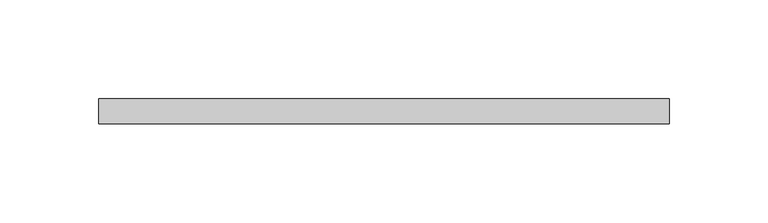
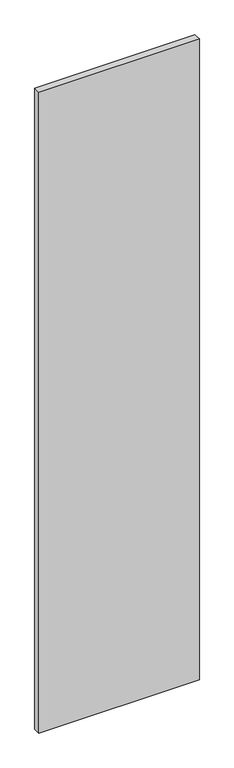
"""IFC4 building model written with IfcOpenShell, lengths in millimetres: proxy geometry, Inner panel:Inner panel:1:Inner panel:1 : Inner panel:Inner panel:300324:300043:Inner panel:1:Inner panel:1 : Inner panel:Inner panel:300324:300043 : Inner panel:Inner panel:1:Inner panel:1 : Inner panel:Inner panel:300324:300043:30 : Inner panel:Inner panel:1:Inner panel:1 : Inner panel:Inner panel:300324:300043:Inner panel:1:Inner panel:1 : Inner panel:Inner panel:300324:300043 : Inner panel:Inner panel:1:Inner panel:1 : Inner panel:Inner panel:300324:300043:300031."""

from ifc_helpers import new_model, si_unit, frame, origin, place, context, project, spatial, polyline, outline, extrude, source, transform, mapped, element, save


def generic_models_07b13941(model_context):
    return source(origin(), model_context, "Body", "SweptSolid", [
        extrude(outline(polyline([(560352.9617239, -579000.6913841), (560641.8867239, -579000.6913841), (560641.8867239, -579013.3913841), (560352.9617239, -579013.3913841), (560352.9617239, -579000.6913841)])), frame((0.0, 0.0, 4946.65), z_axis=(0.0, 0.0, 1.0), x_axis=(1.0, 0.0, 0.0)), (0.0, 0.0, 1.0), 1219.2),
    ])


if __name__ == "__main__":
    model = new_model("IFC4")
    model_context = context("Model", 3, world=origin())
    ifc_project = project(units=[si_unit("LENGTHUNIT", "METRE", prefix="MILLI")], contexts=[model_context])
    site = spatial("IfcSite", under=ifc_project)
    building = spatial("IfcBuilding", under=site)
    placement = place(None, origin())
    generic_models_shape = generic_models_07b13941(model_context)
    element("IfcBuildingElementProxy", 1, Name="Inner panel:Inner panel:1:Inner panel:1 : Inner panel:Inner panel:300324:300043:Inner panel:1:Inner panel:1 : Inner panel:Inner panel:300324:300043 : Inner panel:Inner panel:1:Inner panel:1 : Inner panel:Inner panel:300324:300043:30 : Inner panel:Inner panel:1:Inner panel:1 : Inner panel:Inner panel:300324:300043:Inner panel:1:Inner panel:1 : Inner panel:Inner panel:300324:300043 : Inner panel:Inner panel:1:Inner panel:1 : Inner panel:Inner panel:300324:300043:300031", ObjectType="Inner panel:Inner panel:1:Inner panel:1 : Inner panel:Inner panel:300324:300043:Inner panel:1:Inner panel:1 : Inner panel:Inner panel:300324:300043 : Inner panel:Inner panel:1:Inner panel:1 : Inner panel:Inner panel:300324:300043:30 : Inner panel:Inner panel:1:Inner panel:1 : Inner panel:Inner panel:300324:300043:Inner panel:1:Inner panel:1 : Inner panel:Inner panel:300324:300043 : Inner panel:Inner panel:1:Inner panel:1 : Inner panel:Inner panel:300324:300043:300031", at=placement, inside=building, context=model_context, shape_type="MappedRepresentation", body=[
        mapped(generic_models_shape, transform((0.0, 0.0, 0.0), x_axis=(1.0, 0.0, 0.0), y_axis=(0.0, 1.0, 0.0), z_axis=(0.0, 0.0, 1.0))),
    ])
    save(model, "model.ifc")

# Revit data of these elements
# Type "Inner panel:Inner panel:1:Inner panel:1 : Inner panel:Inner panel:300324:300043:Inner panel:1:Inner panel:1 : Inner panel:Inner panel:300324:300043 : Inner panel:Inner panel:1:Inner panel:1 : Inner panel:Inner panel:300324:300043:30 : Inner panel:Inner panel:1:Inner panel:1 : Inner panel:Inner panel:300324:300043:Inner panel:1:Inner panel:1 : Inner panel:Inner panel:300324:300043 : Inner panel:Inner panel:1:Inner panel:1 : Inner panel:Inner panel:300324:300043:300031"
#   NameOverride = "Inner panel:Inner panel:1:Inner panel:1 : Inner panel:Inner panel:300324:300043:Inner panel:1:Inner panel:1 : Inner panel:Inner panel:300324:300043 : Inner panel:Inner panel:1:Inner panel:1 : Inner panel:Inner panel:300324:300043:300031"
#   ObjectTypeOverride = "Inner panel:1:Inner panel:1 : Inner panel:Inner panel:300324:300043 : Inner panel:Inner panel:1:Inner panel:1 : Inner panel:Inner panel:300324:300043"
#   Reference = "Inner panel"
#   Tag = "300031"
# Element 1 (IfcBuildingElementProxy, "Inner panel:Inner panel:1:Inner panel:1 : Inner panel:Inner panel:300324:300043:Inner panel:1:Inner panel:1 : Inner panel:Inner panel:300324:300043 : Inner panel:Inner panel:1:Inner panel:1 : Inner panel:Inner panel:300324:300043:30 : Inner panel:Inner panel:1:Inner panel:1 : Inner panel:Inner panel:300324:300043:Inner panel:1:Inner panel:1 : Inner panel:Inner panel:300324:300043 : Inner panel:Inner panel:1:Inner panel:1 : Inner panel:Inner panel:300324:300043:300031")
#   Materials on its faces: "1/2\" FIBERGLASS MAT GYPSUM PANELS"
# Materials
#   "1/2\" FIBERGLASS MAT GYPSUM PANELS": class "Generic", colour RGB 171 170 168, transparency 0, Description = "Gypsum Wall Board", Cost = 0
